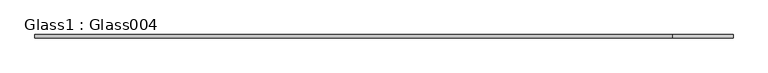
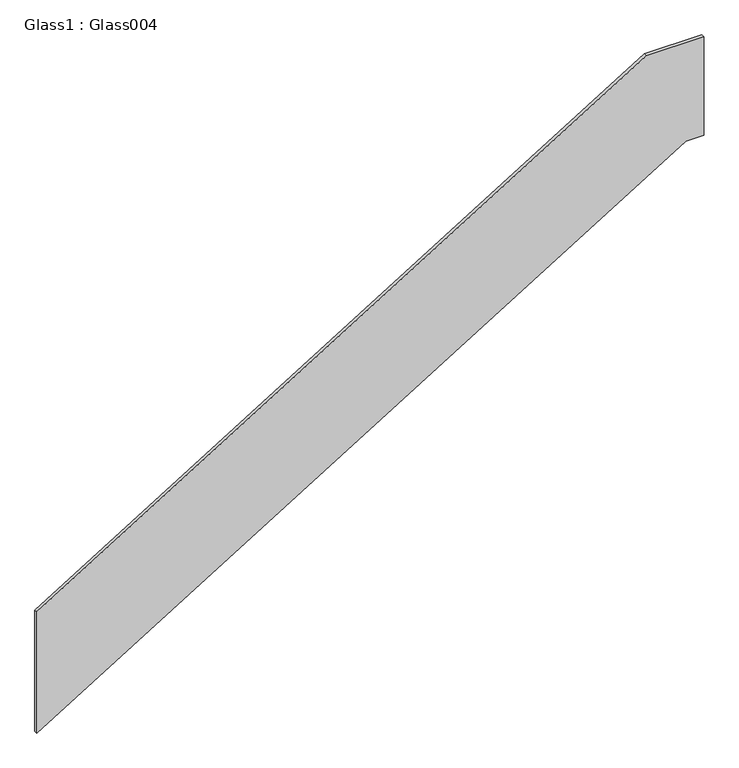
"""IFC4 building model written with IfcOpenShell, lengths in millimetres: proxy geometry, Glass1 : Glass004."""

from ifc_helpers import new_model, si_unit, frame, origin, place, context, project, spatial, polyline, outline, extrude, source, transform, mapped, element, save


def glass1_glass004_3046ee41(model_context):
    return source(origin(), model_context, "Body", "SweptSolid", [
        extrude(outline(polyline([(38035.9266566, 4990.3637308), (37022.6954344, 4990.3637308), (40173.1410997, 10124.4233335), (40173.1410997, 10267.8101348), (40995.0266566, 10267.8101348), (40995.0266566, 9812.6007679), (38035.9266566, 4990.3637308)])), frame((0.0, 1934.5461961, 0.0), z_axis=(0.0, 1.0, 0.0), x_axis=(0.0, 0.0, 1.0)), (0.0, 0.0, 1.0), 25.6840222),
    ])


if __name__ == "__main__":
    model = new_model("IFC4")
    model_context = context("Model", 3, world=origin())
    ifc_project = project(units=[si_unit("LENGTHUNIT", "METRE", prefix="MILLI")], contexts=[model_context])
    site = spatial("IfcSite", under=ifc_project)
    building = spatial("IfcBuilding", under=site)
    placement = place(None, origin())
    glass1_glass004_shape = glass1_glass004_3046ee41(model_context)
    element("IfcBuildingElementProxy", 1, Name="Glass1 : Glass004", ObjectType="Glass1 : Glass004", at=placement, inside=building, context=model_context, shape_type="MappedRepresentation", body=[
        mapped(glass1_glass004_shape, transform((0.0, 0.0, 0.0), x_axis=(1.0, 0.0, 0.0), y_axis=(0.0, 1.0, 0.0), z_axis=(0.0, 0.0, 1.0))),
    ])
    save(model, "model.ifc")

# Revit data of these elements
# Type "Glass1 : Glass004"
#   NameOverride = "Glass004"
# Element 1 (IfcBuildingElementProxy, "Glass1 : Glass004")
#   Materials on its faces: "1/2\" TEMPERED GLASS"
# Materials
#   "1/2\" TEMPERED GLASS": class "Unassigned", colour RGB 191 240 251, transparency 0, Cost = 0
